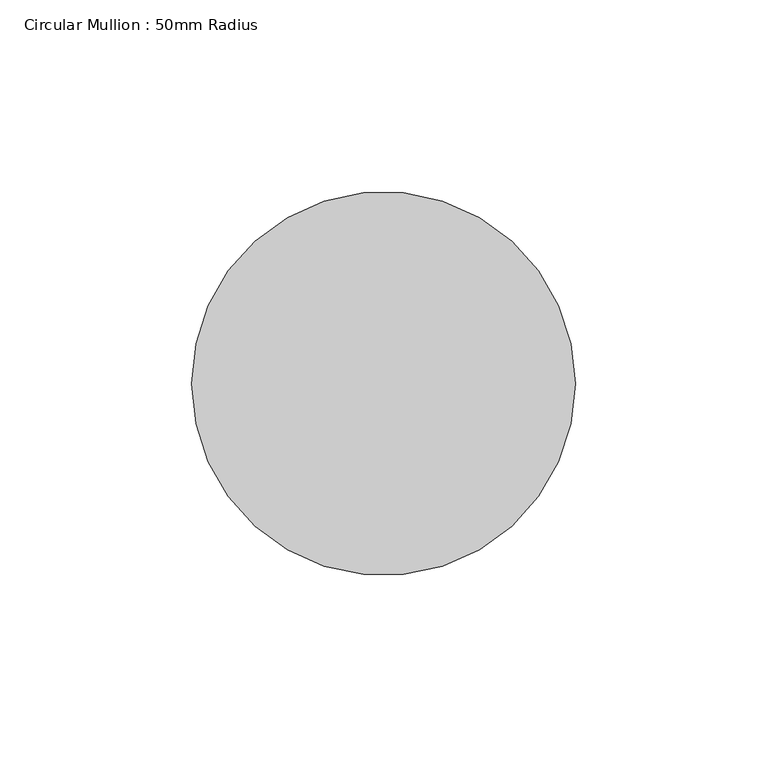
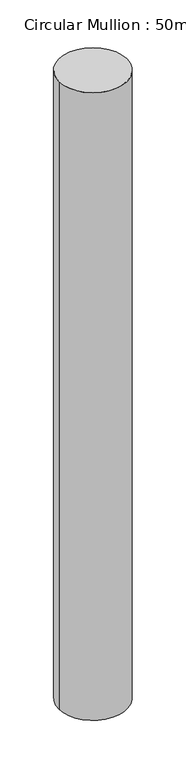
"""IFC4 building model written with IfcOpenShell, lengths in millimetres: member geometry, Circular Mullion : 50mm Radius."""

from ifc_helpers import new_model, si_unit, point, frame, origin, origin_2d, place, context, project, spatial, circle_curve, trimmed, segment, composite_curve, outline, extrude, source, transform, mapped, element, save


def circular_mullion_50mm_radius_6f59e1cc(model_context):
    return source(origin(), model_context, "Body", "SweptSolid", [
        extrude(outline(composite_curve([segment(trimmed(circle_curve(origin_2d(), 50.0), [point((50.0, 0.0))], [point((-50.0, 0.0))], False, "CARTESIAN"), True, "CONTINUOUS"), segment(trimmed(circle_curve(origin_2d(), 50.0), [point((-50.0, 0.0))], [point((50.0, 0.0))], False, "CARTESIAN"), True, "CONTINUOUS")], self_intersect=False)), frame((0.0, 0.0, -972.9002294), z_axis=(0.0, 0.0, 1.0), x_axis=(1.0, 0.0, 0.0)), (0.0, 0.0, 1.0), 972.9002294),
    ])


if __name__ == "__main__":
    model = new_model("IFC4")
    model_context = context("Model", 3, world=origin())
    ifc_project = project(units=[si_unit("LENGTHUNIT", "METRE", prefix="MILLI")], contexts=[model_context])
    site = spatial("IfcSite", under=ifc_project)
    building = spatial("IfcBuilding", under=site)
    placement = place(None, origin())
    circular_mullion_50mm_radius_shape = circular_mullion_50mm_radius_6f59e1cc(model_context)
    element("IfcMember", 1, ObjectType="Circular Mullion : 50mm Radius", at=placement, inside=building, context=model_context, shape_type="MappedRepresentation", body=[
        mapped(circular_mullion_50mm_radius_shape, transform((0.0, 0.0, 0.0), x_axis=(1.0, 0.0, 0.0), y_axis=(0.0, 1.0, 0.0), z_axis=(0.0, 0.0, 1.0))),
    ])
    save(model, "model.ifc")

# Revit data of these elements
# Type "Circular Mullion : 50mm Radius"
#   built-in parameter 1007350 = 0.164042 (stored number, unit not read)
# Element 1 (IfcMember, "Circular Mullion : 50mm Radius")
#   Materials on its faces: "Aluminium"
# Materials
#   "Aluminium": class "Metal", colour RGB 247 247 247, transparency 0, Description = "Aluminium 6061", Cost = 0
